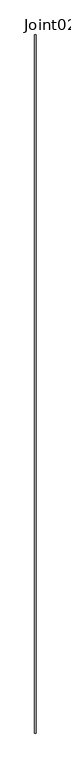
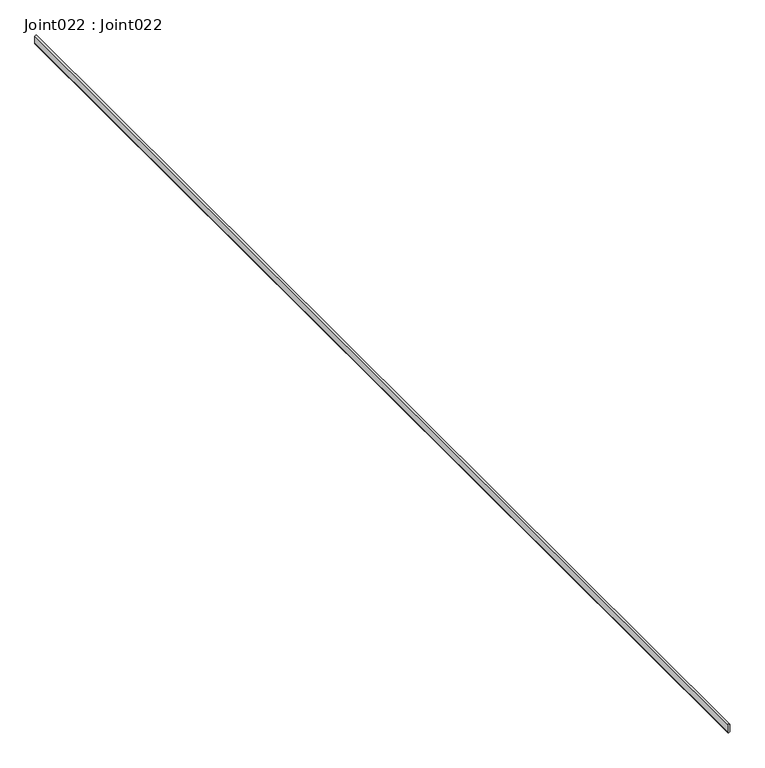
"""IFC4 building model written with IfcOpenShell, lengths in millimetres: proxy geometry, Joint022 : Joint022."""

from ifc_helpers import new_model, si_unit, point, frame, frame_2d, origin, place, context, project, spatial, polyline, circle_curve, trimmed, segment, composite_curve, outline, extrude, source, transform, mapped, element, save


def joint022_joint022_e8a83f9e(model_context):
    return source(origin(), model_context, "Body", "SweptSolid", [
        extrude(outline(composite_curve([segment(polyline([(40205.3911133, -7050.1630859), (40193.3164063, -7050.1630859)]), True, "CONTINUOUS"), segment(trimmed(circle_curve(frame_2d((40193.3164063, -7048.3974609)), 1.765625), [point((40193.3164063, -7050.1630859))], [point((40193.3164063, -7046.6318359))], False, "CARTESIAN"), True, "CONTINUOUS"), segment(polyline([(40193.3164063, -7046.6318359), (40205.3911133, -7046.6318359)]), True, "CONTINUOUS"), segment(trimmed(circle_curve(frame_2d((40205.3911133, -7048.3974609)), 1.765625), [point((40205.3911133, -7046.6318359))], [point((40205.3911133, -7050.1630859))], False, "CARTESIAN"), True, "CONTINUOUS")], self_intersect=False)), frame((0.0, 7982.1531721, 0.0), z_axis=(0.0, 1.0, 0.0), x_axis=(0.0, 0.0, 1.0)), (0.0, 0.0, 1.0), 2000.0),
    ])


if __name__ == "__main__":
    model = new_model("IFC4")
    model_context = context("Model", 3, world=origin())
    ifc_project = project(units=[si_unit("LENGTHUNIT", "METRE", prefix="MILLI")], contexts=[model_context])
    site = spatial("IfcSite", under=ifc_project)
    building = spatial("IfcBuilding", under=site)
    placement = place(None, origin())
    joint022_joint022_shape = joint022_joint022_e8a83f9e(model_context)
    element("IfcBuildingElementProxy", 1, Name="Joint022 : Joint022", ObjectType="Joint022 : Joint022", at=placement, inside=building, context=model_context, shape_type="MappedRepresentation", body=[
        mapped(joint022_joint022_shape, transform((0.0, 0.0, 0.0), x_axis=(1.0, 0.0, 0.0), y_axis=(0.0, 1.0, 0.0), z_axis=(0.0, 0.0, 1.0))),
    ])
    save(model, "model.ifc")

# Revit data of these elements
# Type "Joint022 : Joint022"
#   NameOverride = "Joint022"
# Element 1 (IfcBuildingElementProxy, "Joint022 : Joint022")
#   Materials on its faces: "SILICON JOINT"
# Materials
#   "SILICON JOINT": class "Unassigned", colour RGB 150 184 127, transparency 0
